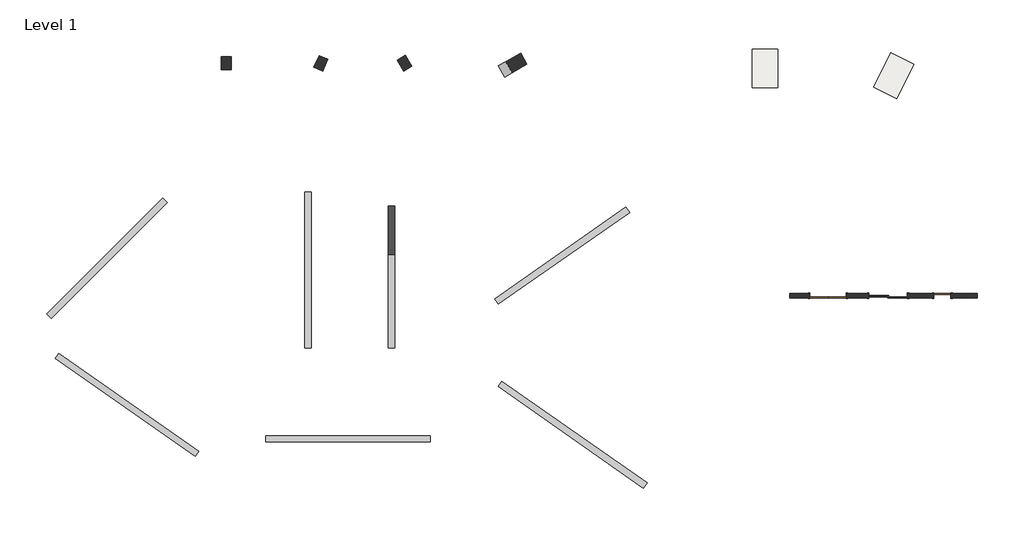
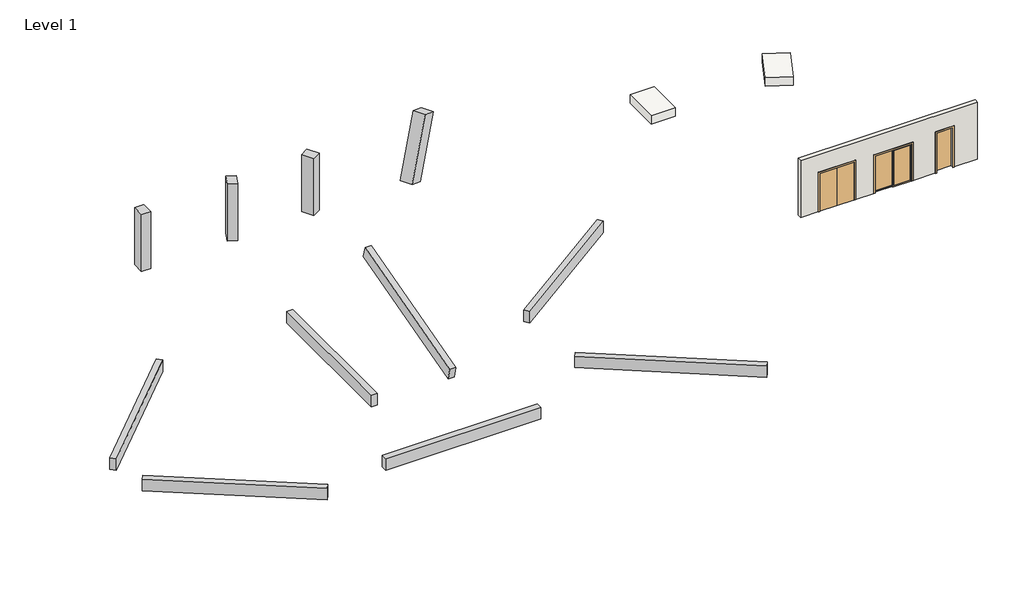
# One storey: 7 beams, 4 columns, 3 doors, 2 slabs, 1 wall.
"""IFC4 building model written with IfcOpenShell, lengths in millimetres."""

import ifcopenshell
import ifcopenshell.guid

model = None  # the IFC model being written
_history = None  # IfcOwnerHistory: only IFC2X3 demands one
_inside = {}  # id of a spatial element -> (the spatial element, [elements in it])
_under = {}  # id of a project, library or spatial element -> (it, [spatial elements below it])
_declared = {}  # id of a project -> (the project, [libraries it declares])
_typed = {}  # id of a type object -> (the type object, [elements of that type])
_made_of = {}  # id of a material, layer set ... -> (it, [elements and type objects made of it])


def new_model(schema):
    """Start an empty IFC model of exactly this schema.

    Asked for "IFC4X3", IfcOpenShell would pick the latest addendum, in which some entities
    have other attributes; the version numbers below select the first issue.
    IFC2X3 requires an IfcOwnerHistory on every rooted entity: one is made here for all.
    """
    global model, _history
    if schema == "IFC4X3":
        model = ifcopenshell.file(schema_version=(4, 3, 0, 0))
    else:
        model = ifcopenshell.file(schema=schema)
    _inside.clear()
    _under.clear()
    _declared.clear()
    _typed.clear()
    _made_of.clear()
    _history = None
    if model.schema == "IFC2X3":
        org = make("IfcOrganization", Name="unknown")
        user = make(
            "IfcPersonAndOrganization",
            ThePerson=make("IfcPerson", FamilyName="unknown"),
            TheOrganization=org,
        )
        app = make(
            "IfcApplication",
            ApplicationDeveloper=org,
            Version="unknown",
            ApplicationFullName="unknown",
            ApplicationIdentifier="unknown",
        )
        _history = make(
            "IfcOwnerHistory",
            OwningUser=user,
            OwningApplication=app,
            ChangeAction="ADDED",
            CreationDate=0,
        )
    return model


def make(cls, **values):
    """One entity of the class cls with the attributes given. An attribute that is None is left unset."""
    return model.create_entity(
        cls, **{name: value for name, value in values.items() if value is not None}
    )


def rooted(cls, **values):
    """An entity with a GlobalId (a new one), such as an element, a storey or a relation."""
    return make(cls, GlobalId=ifcopenshell.guid.new(), OwnerHistory=_history, **values)


def si_unit(unit_type, name, prefix=None):
    """IfcSIUnit, for example si_unit("LENGTHUNIT", "METRE", prefix="MILLI")."""
    return make("IfcSIUnit", UnitType=unit_type, Prefix=prefix, Name=name)


def assignment(units):
    """IfcUnitAssignment: the units of a project."""
    return None if units is None else make("IfcUnitAssignment", Units=units)


def point(xyz):
    """IfcCartesianPoint."""
    return None if xyz is None else make("IfcCartesianPoint", Coordinates=xyz)


def direction(xyz):
    """IfcDirection."""
    return None if xyz is None else make("IfcDirection", DirectionRatios=xyz)


def frame(location, z_axis=None, x_axis=None):
    """IfcAxis2Placement3D, a coordinate frame: its origin and axes. An axis left out is left unset."""
    return make(
        "IfcAxis2Placement3D",
        Location=point(location),
        Axis=direction(z_axis),
        RefDirection=direction(x_axis),
    )


def origin():
    """The frame at (0, 0, 0) with its axes left unset."""
    return frame((0.0, 0.0, 0.0))


def origin_with_axes():
    """The frame at (0, 0, 0) with the z axis (0, 0, 1) and the x axis (1, 0, 0) written out."""
    return frame((0.0, 0.0, 0.0), z_axis=(0.0, 0.0, 1.0), x_axis=(1.0, 0.0, 0.0))


def place(relative_to, where):
    """IfcLocalPlacement: puts the frame where relative to a parent placement (None: the world)."""
    return make(
        "IfcLocalPlacement", PlacementRelTo=relative_to, RelativePlacement=where
    )


def context(
    kind, dimensions, precision=None, world=None, true_north=None, identifier=None
):
    """IfcGeometricRepresentationContext, for example the 3D "Model" context."""
    return make(
        "IfcGeometricRepresentationContext",
        ContextIdentifier=identifier,
        ContextType=kind,
        CoordinateSpaceDimension=dimensions,
        Precision=precision,
        WorldCoordinateSystem=world,
        TrueNorth=true_north,
    )


def project(units=None, contexts=None):
    """IfcProject with its units and contexts."""
    return rooted(
        "IfcProject",
        Name="project",
        RepresentationContexts=contexts,
        UnitsInContext=assignment(units),
    )


def spatial(cls, under=None, at=None, **own):
    """A site, building, storey or space (cls), placed at a placement, below another one or the project."""
    s = rooted(cls, ObjectPlacement=at, **own)
    if under is not None:
        _under.setdefault(under.id(), (under, []))[1].append(s)
    return s


def polyline(points):
    """IfcPolyline through the points."""
    return make("IfcPolyline", Points=[point(p) for p in points])


def outline(outer, holes=None, kind="AREA"):
    """IfcArbitraryClosedProfileDef: a profile drawn as a closed curve; with holes, ...WithVoids."""
    if holes is None:
        return make("IfcArbitraryClosedProfileDef", ProfileType=kind, OuterCurve=outer)
    return make(
        "IfcArbitraryProfileDefWithVoids",
        ProfileType=kind,
        OuterCurve=outer,
        InnerCurves=holes,
    )


def extrude(swept, where, along, depth):
    """IfcExtrudedAreaSolid: the profile swept, set in the frame where, extruded along a direction by depth."""
    return make(
        "IfcExtrudedAreaSolid",
        SweptArea=swept,
        Position=where,
        ExtrudedDirection=direction(along),
        Depth=depth,
    )


def shape(context_of_items, identifier, shape_type, items):
    """IfcShapeRepresentation: the items that make up one representation, for example the "Body"."""
    return make(
        "IfcShapeRepresentation",
        ContextOfItems=context_of_items,
        RepresentationIdentifier=identifier,
        RepresentationType=shape_type,
        Items=items,
    )


def source(mapping_origin, context_of_items, identifier, shape_type, items):
    """IfcRepresentationMap: a shape defined once, which mapped items show again and again."""
    return make(
        "IfcRepresentationMap",
        MappingOrigin=mapping_origin,
        MappedRepresentation=shape(context_of_items, identifier, shape_type, items),
    )


def transform(
    local_origin,
    x_axis=None,
    y_axis=None,
    z_axis=None,
    scale=None,
    scale2=None,
    scale3=None,
    uniform=True,
):
    """IfcCartesianTransformationOperator3D, or its non-uniform kind. x_axis, y_axis, z_axis: its Axis1, 2, 3."""
    if uniform:
        return make(
            "IfcCartesianTransformationOperator3D",
            Axis1=direction(x_axis),
            Axis2=direction(y_axis),
            LocalOrigin=point(local_origin),
            Scale=scale,
            Axis3=direction(z_axis),
        )
    return make(
        "IfcCartesianTransformationOperator3DnonUniform",
        Axis1=direction(x_axis),
        Axis2=direction(y_axis),
        LocalOrigin=point(local_origin),
        Scale=scale,
        Axis3=direction(z_axis),
        Scale2=scale2,
        Scale3=scale3,
    )


def mapped(mapping_source, mapping_target):
    """IfcMappedItem: shows the shape of a source again, moved by a transform."""
    return make(
        "IfcMappedItem", MappingSource=mapping_source, MappingTarget=mapping_target
    )


def made_of(thing, what):
    """Note that an element or type object is made of a material, layer set ...; save() writes the relation."""
    if what is not None:
        _made_of.setdefault(what.id(), (what, []))[1].append(thing)
    return thing


def element(
    cls,
    number,
    at=None,
    inside=None,
    cuts=None,
    type_object=None,
    material=None,
    context=None,
    identifier="Body",
    shape_type=None,
    held_by="IfcProductDefinitionShape",
    body=None,
    shapes=None,
    **own,
):
    """One element of the class cls, such as IfcWall. Its Tag is "e" and its number.

    at: its placement. inside: the storey or other place that contains it. cuts: it is an
    opening in that element (IfcRelVoidsElement). A single representation is given by context,
    identifier, shape_type and body (its items); several are given by shapes. held_by: the class
    of the entity that holds the representations. save() writes the other relations.
    """
    e = rooted(cls, Tag="e%d" % number, ObjectPlacement=at, **own)
    if body is not None:
        shapes = [shape(context, identifier, shape_type, body)]
    if shapes is not None:
        e.Representation = make(held_by, Representations=shapes)
    if inside is not None:
        _inside.setdefault(inside.id(), (inside, []))[1].append(e)
    if cuts is not None:
        rooted(
            "IfcRelVoidsElement", RelatingBuildingElement=cuts, RelatedOpeningElement=e
        )
    if type_object is not None:
        _typed.setdefault(type_object.id(), (type_object, []))[1].append(e)
    return made_of(e, material)


def aggregate(whole, parts):
    """IfcRelAggregates: a whole, such as a stair, and the parts it consists of."""
    return rooted("IfcRelAggregates", RelatingObject=whole, RelatedObjects=parts)


def save(model, path):
    """Write the relations noted so far, then the file.

    IfcRelAggregates (storeys below a building ...), IfcRelContainedInSpatialStructure (elements
    in a storey), IfcRelDefinesByType, IfcRelAssociatesMaterial and IfcRelDeclares: one each for
    every whole, place, type object, material and project.
    """
    for whole, parts in _under.values():
        aggregate(whole, parts)
    for where, things in _inside.values():
        rooted(
            "IfcRelContainedInSpatialStructure",
            RelatedElements=things,
            RelatingStructure=where,
        )
    for kind, things in _typed.values():
        rooted("IfcRelDefinesByType", RelatedObjects=things, RelatingType=kind)
    for what, things in _made_of.values():
        rooted("IfcRelAssociatesMaterial", RelatedObjects=things, RelatingMaterial=what)
    for by, libraries in _declared.values():
        rooted("IfcRelDeclares", RelatingContext=by, RelatedDefinitions=libraries)
    model.write(path)


def concrete_rectangular_beam_300_x_600mm_0e8e550c(model_context):
    return source(origin(), model_context, "Body", "SweptSolid", [
        extrude(outline(polyline([(4000.0, 150.0), (4000.0, -150.0), (-4000.0, -150.0), (-4000.0, 150.0), (4000.0, 150.0)])), frame((0.0, 0.0, -300.0), z_axis=(0.0, 0.0, 1.0), x_axis=(1.0, 0.0, 0.0)), (0.0, 0.0, 1.0), 600.0),
    ])


def concrete_rectangular_beam_300_x_600mm_526adf45(model_context):
    return source(origin(), model_context, "Body", "SweptSolid", [
        extrude(outline(polyline([(3850.0, 150.0), (3850.0, -150.0), (-3850.0, -150.0), (-3850.0, 150.0), (3850.0, 150.0)])), frame((0.0, 0.0, -300.0), z_axis=(0.0, 0.0, 1.0), x_axis=(1.0, 0.0, 0.0)), (0.0, 0.0, 1.0), 600.0),
    ])


def concrete_rectangular_beam_300_x_600mm_2f98737b(model_context):
    return source(origin(), model_context, "Body", "SweptSolid", [
        extrude(outline(polyline([(3650.0, 150.0), (3650.0, -150.0), (-3650.0, -150.0), (-3650.0, 150.0), (3650.0, 150.0)])), frame((0.0, 0.0, -300.0), z_axis=(0.0, 0.0, 1.0), x_axis=(1.0, 0.0, 0.0)), (0.0, 0.0, 1.0), 600.0),
    ])


def concrete_rectangular_beam_300_x_600mm_b31908cc(model_context):
    return source(origin(), model_context, "Body", "SweptSolid", [
        extrude(outline(polyline([(3750.0, 150.0), (3750.0, -150.0), (-3750.0, -150.0), (-3750.0, 150.0), (3750.0, 150.0)])), frame((0.0, 0.0, -300.0), z_axis=(0.0, 0.0, 1.0), x_axis=(1.0, 0.0, 0.0)), (0.0, 0.0, 1.0), 600.0),
    ])


def concrete_rectangular_beam_300_x_600mm_b1d28744(model_context):
    return source(origin(), model_context, "Body", "SweptSolid", [
        extrude(outline(polyline([(4150.0, 150.0), (4150.0, -150.0), (-4150.0, -150.0), (-4150.0, 150.0), (4150.0, 150.0)])), frame((0.0, 0.0, -300.0), z_axis=(0.0, 0.0, 1.0), x_axis=(1.0, 0.0, 0.0)), (0.0, 0.0, 1.0), 600.0),
    ])


def concrete_rectangular_beam_300_x_600mm_07bb940a(model_context):
    return source(origin(), model_context, "Body", "SweptSolid", [
        extrude(outline(polyline([(3784.507894, 150.0), (3784.507894, -150.0), (-3784.507894, -150.0), (-3784.507894, 150.0), (3784.507894, 150.0)])), frame((0.0, 0.0, -300.0), z_axis=(0.0, 0.0, 1.0), x_axis=(1.0, 0.0, 0.0)), (0.0, 0.0, 1.0), 600.0),
    ])


def concrete_rectangular_column_450_x_600mm_2b408faa(model_context):
    return source(origin(), model_context, "Body", "SweptSolid", [
        extrude(outline(polyline([(225.0, 300.0), (225.0, -300.0), (-225.0, -300.0), (-225.0, 300.0), (225.0, 300.0)])), origin_with_axes(), (0.0, 0.0, 1.0), 3000.0),
    ])


def m_door_double_flush_panel_1700_x_2000mm_deeb3825(model_context):
    return source(origin(), model_context, "Body", "SweptSolid", [
        extrude(outline(polyline([(2000.0, -850.0), (2000.0, 850.0), (0.0, 850.0), (0.0, 930.0), (2080.0, 930.0), (2080.0, -930.0), (0.0, -930.0), (0.0, -850.0), (2000.0, -850.0)])), frame((0.0, -125.0, 0.0), z_axis=(0.0, 1.0, 0.0), x_axis=(0.0, 0.0, 1.0)), (0.0, 0.0, 1.0), 25.0),
        extrude(outline(polyline([(2000.0, -850.0), (2000.0, 850.0), (0.0, 850.0), (0.0, 930.0), (2080.0, 930.0), (2080.0, -930.0), (0.0, -930.0), (0.0, -850.0), (2000.0, -850.0)])), frame((0.0, 100.0, 0.0), z_axis=(0.0, 1.0, 0.0), x_axis=(0.0, 0.0, 1.0)), (0.0, 0.0, 1.0), 25.0),
        extrude(outline(polyline([(0.0, 100.0), (850.0, 100.0), (850.0, 50.0), (0.0, 50.0), (0.0, 100.0)])), origin_with_axes(), (0.0, 0.0, 1.0), 2000.0),
        extrude(outline(polyline([(-850.0, 100.0), (0.0, 100.0), (0.0, 50.0), (-850.0, 50.0), (-850.0, 100.0)])), origin_with_axes(), (0.0, 0.0, 1.0), 2000.0),
    ])


def m_door_double_sliding_1800_x_1950mm_ddb0fbbc(model_context):
    return source(origin(), model_context, "Body", "SweptSolid", [
        extrude(outline(polyline([(0.0, -980.0), (0.0, -900.0), (1950.0, -900.0), (1950.0, 900.0), (0.0, 900.0), (0.0, 980.0), (2030.0, 980.0), (2030.0, -980.0), (0.0, -980.0)])), frame((0.0, 2.0, 0.0), z_axis=(0.0, 1.0, 0.0), x_axis=(0.0, 0.0, 1.0)), (0.0, 0.0, 1.0), 25.0),
        extrude(outline(polyline([(0.0, 980.0), (2030.0, 980.0), (2030.0, -980.0), (0.0, -980.0), (0.0, -900.0), (1950.0, -900.0), (1950.0, 900.0), (0.0, 900.0), (0.0, 980.0)])), frame((0.0, 227.0, 0.0), z_axis=(0.0, 1.0, 0.0), x_axis=(0.0, 0.0, 1.0)), (0.0, 0.0, 1.0), 25.0),
        extrude(outline(polyline([(1950.0, -25.0), (0.0, -25.0), (0.0, 900.0), (1950.0, 900.0), (1950.0, -25.0)]), holes=[polyline([(1900.0, 25.0), (1900.0, 850.0), (50.0, 850.0), (50.0, 25.0), (1900.0, 25.0)])]), frame((0.0, 127.0, 0.0), z_axis=(0.0, 1.0, 0.0), x_axis=(0.0, 0.0, 1.0)), (0.0, 0.0, 1.0), 50.0),
        extrude(outline(polyline([(1950.0, 25.0), (1950.0, -900.0), (0.0, -900.0), (0.0, 25.0), (1950.0, 25.0)]), holes=[polyline([(1900.0, -25.0), (50.0, -25.0), (50.0, -850.0), (1900.0, -850.0), (1900.0, -25.0)])]), frame((0.0, 177.0, 0.0), z_axis=(0.0, 1.0, 0.0), x_axis=(0.0, 0.0, 1.0)), (0.0, 0.0, 1.0), 50.0),
        extrude(outline(polyline([(25.0, 155.175), (850.0, 155.175), (850.0, 148.825), (25.0, 148.825), (25.0, 155.175)])), frame((0.0, 0.0, 50.0), z_axis=(0.0, 0.0, 1.0), x_axis=(1.0, 0.0, 0.0)), (0.0, 0.0, 1.0), 1850.0),
        extrude(outline(polyline([(-25.0, 200.025), (-850.0, 200.025), (-850.0, 206.375), (-25.0, 206.375), (-25.0, 200.025)])), frame((0.0, 0.0, 50.0), z_axis=(0.0, 0.0, 1.0), x_axis=(1.0, 0.0, 0.0)), (0.0, 0.0, 1.0), 1850.0),
    ])


def m_door_single_panel_800_x_2100mm_e6cd55ec(model_context):
    return source(origin(), model_context, "Body", "SweptSolid", [
        extrude(outline(polyline([(400.0, 50.0), (-400.0, 50.0), (-400.0, 100.0), (400.0, 100.0), (400.0, 50.0)])), origin_with_axes(), (0.0, 0.0, 1.0), 2100.0),
        extrude(outline(polyline([(2176.2, -476.2), (0.0, -476.2), (0.0, -400.0), (2100.0, -400.0), (2100.0, 400.0), (0.0, 400.0), (0.0, 476.2), (2176.2, 476.2), (2176.2, -476.2)])), frame((0.0, 100.0, 0.0), z_axis=(0.0, 1.0, 0.0), x_axis=(0.0, 0.0, 1.0)), (0.0, 0.0, 1.0), 25.0),
        extrude(outline(polyline([(2176.2, 476.2), (2176.2, -476.2), (0.0, -476.2), (0.0, -400.0), (2100.0, -400.0), (2100.0, 400.0), (0.0, 400.0), (0.0, 476.2), (2176.2, 476.2)])), frame((0.0, -125.0, 0.0), z_axis=(0.0, 1.0, 0.0), x_axis=(0.0, 0.0, 1.0)), (0.0, 0.0, 1.0), 25.0),
    ])


def m_footing_rectangular_1800_x_1200_x_450mm_16ba7ea5(model_context):
    return source(origin(), model_context, "Body", "SweptSolid", [
        extrude(outline(polyline([(600.0, 900.0), (600.0, -900.0), (-600.0, -900.0), (-600.0, 900.0), (600.0, 900.0)])), frame((0.0, 0.0, -450.0), z_axis=(0.0, 0.0, 1.0), x_axis=(1.0, 0.0, 0.0)), (0.0, 0.0, 1.0), 450.0),
    ])


model = new_model("IFC4")

# Units and contexts
model_context = context("Model", 3, world=origin())
ifc_project = project(units=[si_unit("LENGTHUNIT", "METRE", prefix="MILLI")], contexts=[model_context])

# Site, building, storey
site = spatial("IfcSite", under=ifc_project)
building = spatial("IfcBuilding", under=site)
storey = spatial("IfcBuildingStorey", under=building, Name="Level 1", Elevation=0.0)

# Beams
placement = place(None, origin())
concrete_rectangular_beam_300_x_600mm_shape = concrete_rectangular_beam_300_x_600mm_0e8e550c(model_context)
element("IfcBeam", 1, ObjectType="Concrete-Rectangular Beam : 300 x 600mm", at=placement, inside=storey, context=model_context, shape_type="MappedRepresentation", body=[
    mapped(concrete_rectangular_beam_300_x_600mm_shape, transform((-9145.2085867, -16555.4936157, -300.0), x_axis=(0.8191520442889902, -0.5735764363510482, 0.0), y_axis=(0.5735764363510482, 0.8191520442889902, 0.0), z_axis=(0.0, 0.0, 1.0))),
])
concrete_rectangular_beam_300_x_600mm_2_shape = concrete_rectangular_beam_300_x_600mm_526adf45(model_context)
element("IfcBeam", 2, ObjectType="Concrete-Rectangular Beam : 300 x 600mm", at=placement, inside=storey, context=model_context, shape_type="MappedRepresentation", body=[
    mapped(concrete_rectangular_beam_300_x_600mm_2_shape, transform((-10087.4940608, -9679.7277386, -300.0), x_axis=(0.7071067811865487, 0.7071067811865464, 0.0), y_axis=(-0.7071067811865464, 0.7071067811865487, 0.0), z_axis=(0.0, 0.0, 1.0))),
])
element("IfcBeam", 3, ObjectType="Concrete-Rectangular Beam : 300 x 600mm", at=placement, inside=storey, context=model_context, shape_type="MappedRepresentation", body=[
    mapped(concrete_rectangular_beam_300_x_600mm_2_shape, transform((1194.8081303, -18143.0516491, -300.0), x_axis=(1.0, 0.0, 0.0), y_axis=(0.0, 1.0, 0.0), z_axis=(0.0, 0.0, 1.0))),
])
concrete_rectangular_beam_300_x_600mm_3_shape = concrete_rectangular_beam_300_x_600mm_2f98737b(model_context)
element("IfcBeam", 4, ObjectType="Concrete-Rectangular Beam : 300 x 600mm", at=placement, inside=storey, context=model_context, shape_type="MappedRepresentation", body=[
    mapped(concrete_rectangular_beam_300_x_600mm_3_shape, transform((-663.497906, -10225.1317807, -300.0), x_axis=(0.0, 1.0, 0.0), y_axis=(-1.0, 0.0, 0.0), z_axis=(0.0, 0.0, 1.0))),
])
concrete_rectangular_beam_300_x_600mm_4_shape = concrete_rectangular_beam_300_x_600mm_b31908cc(model_context)
element("IfcBeam", 5, ObjectType="Concrete-Rectangular Beam : 300 x 600mm", at=placement, inside=storey, context=model_context, shape_type="MappedRepresentation", body=[
    mapped(concrete_rectangular_beam_300_x_600mm_4_shape, transform((11230.4771438, -9556.8124673, -300.0), x_axis=(-0.8191520442889922, -0.5735764363510455, 0.0), y_axis=(0.5735764363510455, -0.8191520442889922, 0.0), z_axis=(0.0, 0.0, 1.0))),
])
concrete_rectangular_beam_300_x_600mm_5_shape = concrete_rectangular_beam_300_x_600mm_b1d28744(model_context)
element("IfcBeam", 6, ObjectType="Concrete-Rectangular Beam : 300 x 600mm", at=placement, inside=storey, context=model_context, shape_type="MappedRepresentation", body=[
    mapped(concrete_rectangular_beam_300_x_600mm_5_shape, transform((11724.551203, -17950.7315453, -300.0), x_axis=(-0.8191520442889885, 0.5735764363510507, 0.0), y_axis=(-0.5735764363510507, -0.8191520442889885, 0.0), z_axis=(0.0, 0.0, 1.0))),
])
concrete_rectangular_beam_300_x_600mm_6_shape = concrete_rectangular_beam_300_x_600mm_07bb940a(model_context)
element("IfcBeam", 7, ObjectType="Concrete-Rectangular Beam : 300 x 600mm", at=placement, inside=storey, context=model_context, shape_type="MappedRepresentation", body=[
    mapped(concrete_rectangular_beam_300_x_600mm_6_shape, transform((3236.502094, -10145.8612366, 710.6625139), x_axis=(0.0, 0.9644582868368909, 0.2642351470786003), y_axis=(-1.0, 0.0, 0.0), z_axis=(0.0, -0.2642351470786003, 0.9644582868368909))),
])

# Columns
concrete_rectangular_column_450_x_600mm_shape = concrete_rectangular_column_450_x_600mm_2b408faa(model_context)
element("IfcColumn", 8, ObjectType="Concrete-Rectangular-Column : 450 x 600mm", at=placement, inside=storey, context=model_context, shape_type="MappedRepresentation", body=[
    mapped(concrete_rectangular_column_450_x_600mm_shape, transform((-4498.8166129, -540.542419, 0.0), x_axis=(1.0, 0.0, 0.0), y_axis=(0.0, 1.0, 0.0), z_axis=(0.0, 0.0, 1.0))),
])
element("IfcColumn", 9, ObjectType="Concrete-Rectangular-Column : 450 x 600mm", at=placement, inside=storey, context=model_context, shape_type="MappedRepresentation", body=[
    mapped(concrete_rectangular_column_450_x_600mm_shape, transform((-64.8783295, -540.542419, 0.0), x_axis=(0.9135454576425981, -0.40673664307580637, 0.0), y_axis=(0.40673664307580637, 0.9135454576425981, 0.0), z_axis=(0.0, 0.0, 1.0))),
])
element("IfcColumn", 10, ObjectType="Concrete-Rectangular-Column : 450 x 600mm", at=placement, inside=storey, context=model_context, shape_type="MappedRepresentation", body=[
    mapped(concrete_rectangular_column_450_x_600mm_shape, transform((3848.4631718, -540.542419, 0.0), x_axis=(0.8571673007021157, 0.5150380749100485, 0.0), y_axis=(-0.5150380749100485, 0.8571673007021157, 0.0), z_axis=(0.0, 0.0, 1.0))),
])
element("IfcColumn", 11, ObjectType="Concrete-Rectangular-Column : 600 x 750mm", at=placement, inside=storey, context=model_context, shape_type="SweptSolid", body=[
    extrude(outline(polyline([(600.0, 0.0), (600.0, -750.0), (0.0, -750.0), (0.0, 0.0), (600.0, 0.0)])), frame((8541.7495915, -1181.0366975, 130.4944773), z_axis=(0.30136408628102856, 0.17399263633843867, 0.9375000000000002), x_axis=(-0.5000000000000028, 0.866025403784437, 0.0)), (0.0, 0.0, 1.0), 3200.0),
])

# Doors
m_door_double_flush_panel_1700_x_2000mm_shape = m_door_double_flush_panel_1700_x_2000mm_deeb3825(model_context)
element("IfcDoor", 12, ObjectType="M_Door-Double-Flush_Panel : 1700 x 2000mm", at=placement, inside=storey, context=model_context, shape_type="MappedRepresentation", body=[
    mapped(m_door_double_flush_panel_1700_x_2000mm_shape, transform((23681.5621943, -11433.3538056, 0.0), x_axis=(-1.0, 0.0, 0.0), y_axis=(0.0, -1.0, 0.0), z_axis=(0.0, 0.0, 1.0))),
])
m_door_double_sliding_1800_x_1950mm_shape = m_door_double_sliding_1800_x_1950mm_ddb0fbbc(model_context)
element("IfcDoor", 13, ObjectType="M_Door-Double-Sliding : 1800 x 1950mm", at=placement, inside=storey, context=model_context, shape_type="MappedRepresentation", body=[
    mapped(m_door_double_sliding_1800_x_1950mm_shape, transform((26491.5621943, -11306.3538056, 0.0), x_axis=(-1.0, 0.0, 0.0), y_axis=(0.0, -1.0, 0.0), z_axis=(0.0, 0.0, 1.0))),
])
m_door_single_panel_800_x_2100mm_shape = m_door_single_panel_800_x_2100mm_e6cd55ec(model_context)
element("IfcDoor", 14, ObjectType="M_Door-Single-Panel : 800 x 2100mm", at=placement, inside=storey, context=model_context, shape_type="MappedRepresentation", body=[
    mapped(m_door_single_panel_800_x_2100mm_shape, transform((29036.5621943, -11433.3538056, 0.0), x_axis=(1.0, 0.0, 0.0), y_axis=(0.0, 1.0, 0.0), z_axis=(0.0, 0.0, 1.0))),
])

# Slabs
m_footing_rectangular_1800_x_1200_x_450mm_shape = m_footing_rectangular_1800_x_1200_x_450mm_16ba7ea5(model_context)
element("IfcSlab", 15, ObjectType="M_Footing-Rectangular : 1800 x 1200 x 450mm", at=placement, inside=storey, context=model_context, shape_type="MappedRepresentation", body=[
    mapped(m_footing_rectangular_1800_x_1200_x_450mm_shape, transform((20736.502094, -775.1317807, 0.0), x_axis=(1.0, 0.0, 0.0), y_axis=(0.0, 1.0, 0.0), z_axis=(0.0, 0.0, 1.0))),
])
element("IfcSlab", 16, ObjectType="M_Footing-Rectangular : 1800 x 1200 x 450mm", at=placement, inside=storey, context=model_context, shape_type="MappedRepresentation", body=[
    mapped(m_footing_rectangular_1800_x_1200_x_450mm_shape, transform((26762.5678616, -1118.6772691, 0.0), x_axis=(0.898794046299165, -0.4383711467890819, 0.0), y_axis=(0.4383711467890819, 0.898794046299165, 0.0), z_axis=(0.0, 0.0, 1.0))),
])

# Wall
element("IfcWall", 17, ObjectType="Generic - 200mm", at=placement, inside=storey, context=model_context, shape_type="SweptSolid", body=[
    extrude(outline(polyline([(2100.0, 29436.5621943), (0.0, 29436.5621943), (0.0, 30676.5621943), (3000.0, 30676.5621943), (3000.0, 21876.5621943), (0.0, 21876.5621943), (0.0, 22831.5621943), (2000.0, 22831.5621943), (2000.0, 24531.5621943), (0.0, 24531.5621943), (0.0, 25591.5621943), (1950.0, 25591.5621943), (1950.0, 27391.5621943), (0.0, 27391.5621943), (0.0, 28636.5621943), (2100.0, 28636.5621943), (2100.0, 29436.5621943)])), frame((0.0, -11533.3538056, 0.0), z_axis=(0.0, 1.0, 0.0), x_axis=(0.0, 0.0, 1.0)), (0.0, 0.0, 1.0), 200.0),
])

save(model, "model.ifc")

# Revit data of these elements
# Project information
#   Project Issue Date = "Issue Date"
#   Project Status = "Project Status"
#   Client Name = "Owner"
#   Project Address = "Enter address here"
#   Project Name = "Project Name"
#   Project Number = "Project Number"
#   SR Document GUID = "d4a11de3-9f94-4c30-a072-1203588bd18a"
# Type "Concrete-Rectangular Beam : 300 x 600mm"
#   Length [instance default] = 1524 mm
#   b = 300 mm
#   h = 600 mm
#   Structural Material [instance default] = Concrete, Cast-in-Place gray
#   Assembly Code = ""
# Type "Concrete-Rectangular-Column : 450 x 600mm"
#   b = 450 mm
#   h = 600 mm
#   Structural Material [instance default] = none
# Type "Concrete-Rectangular-Column : 600 x 750mm"
#   b = 600 mm
#   h = 750 mm
#   Structural Material [instance default] = none
# Type "M_Door-Double-Flush_Panel : 1700 x 2000mm"
#   Type Mark = "41"
#   Construction Type Id = "DOOR"
#   Assembly Code = "C1020"
#   Analytic Construction = "Wooden"
#   Thickness = 50 mm
#   Thermal Resistance (R) = 0.455703 (m²·K)/W
#   Swing Angle [instance default] = 90.00°
#   Panel Width = 850 mm
#   Heat Transfer Coefficient (U) = 2.19465 W/(m²·K)
#   Height = 2000 mm
#   Trim Projection Ext = 25 mm
#   Trim Projection Int = 25 mm
#   Trim Width = 80 mm
#   Width = 1700 mm
#   Panel Material = Wood - Birch - Solid Stained Light Low Gloss
#   Trim Material = Paint - Sienna
#   Visual Light Transmittance = 0
#   Solar Heat Gain Coefficient = 0
#   Function = (empty or 0)
#   Wall Closure = (empty or 0)
# Type "M_Door-Double-Sliding : 1800 x 1950mm"
#   Type Mark = "42"
#   Construction Type Id = "opn-d45"
#   Assembly Code = "C1020"
#   Analytic Construction = "Wood frame, double glass door "
#   Thickness = 50 mm
#   Thermal Resistance (R) = 0.31964 (m²·K)/W
#   Heat Transfer Coefficient (U) = 3.12872 W/(m²·K)
#   Height = 1950 mm
#   Rail Width = 50 mm
#   Stiles = 50 mm
#   Trim Projection Ext = 25 mm
#   Trim Projection Int = 25 mm
#   Trim Width = 80 mm
#   Width = 1800 mm
#   Glazing = Glass
#   Panel Material = Wood - Birch - Solid Stained Light Low Gloss
#   Trim Material = Paint - Sienna
#   Visual Light Transmittance = 0
#   Solar Heat Gain Coefficient = 0
#   Function = (empty or 0)
#   Wall Closure = (empty or 0)
# Type "M_Door-Single-Panel : 800 x 2100mm"
#   Type Mark = "43"
#   Construction Type Id = "DOOR"
#   Assembly Code = "C1020300"
#   Analytic Construction = "Wooden"
#   Thickness = 50 mm
#   Thermal Resistance (R) = 0.455703 (m²·K)/W
#   Swing Angle [instance default] = 90.00°
#   Heat Transfer Coefficient (U) = 2.19465 W/(m²·K)
#   Height = 2100 mm
#   Trim Projection Ext = 25 mm
#   Trim Projection Int = 25 mm
#   Trim Width = 80 mm
#   Width = 800 mm
#   Panel Material = Wood - Birch - Solid Stained Light Low Gloss
#   Trim Material = Paint - Sienna
#   Visual Light Transmittance = 0
#   Solar Heat Gain Coefficient = 0
#   Function = (empty or 0)
#   Wall Closure = (empty or 0)
# Type "M_Footing-Rectangular : 1800 x 1200 x 450mm"
#   Width = 1200 mm
#   Length = 1800 mm
#   Thickness = 450 mm
#   Structural Material [instance default] = none
#   Assembly Code = ""
# Type "Generic - 200mm"
#   Layers, outside or top first: 200 mm no material (function 1)
# Element 1 (IfcBeam, "Concrete-Rectangular Beam : 300 x 600mm")
#   Mark = "B2"
#   Structural Material = Concrete, Cast-in-Place gray
#   Phase Created = New Construction
#   Materials on its faces: "Concrete, Cast-in-Place gray"
# Element 2 (IfcBeam, "Concrete-Rectangular Beam : 300 x 600mm")
#   Mark = "B1"
#   Structural Material = Concrete, Cast-in-Place gray
#   Phase Created = New Construction
#   Materials on its faces: "Concrete, Cast-in-Place gray"
# Element 3 (IfcBeam, "Concrete-Rectangular Beam : 300 x 600mm")
#   Mark = "B3"
#   Structural Material = Concrete, Cast-in-Place gray
#   Phase Created = New Construction
#   Materials on its faces: "Concrete, Cast-in-Place gray"
# Element 4 (IfcBeam, "Concrete-Rectangular Beam : 300 x 600mm")
#   Mark = "B4"
#   Structural Material = Concrete, Cast-in-Place gray
#   Phase Created = New Construction
#   Materials on its faces: "Concrete, Cast-in-Place gray"
# Element 5 (IfcBeam, "Concrete-Rectangular Beam : 300 x 600mm")
#   Mark = "B6"
#   Structural Material = Concrete, Cast-in-Place gray
#   Phase Created = New Construction
#   Materials on its faces: "Concrete, Cast-in-Place gray"
# Element 6 (IfcBeam, "Concrete-Rectangular Beam : 300 x 600mm")
#   Mark = "B7"
#   Structural Material = Concrete, Cast-in-Place gray
#   Phase Created = New Construction
#   Materials on its faces: "Concrete, Cast-in-Place gray"
# Element 7 (IfcBeam, "Concrete-Rectangular Beam : 300 x 600mm")
#   Mark = "B5"
#   Structural Material = Concrete, Cast-in-Place gray
#   Phase Created = New Construction
#   Materials on its faces: "Concrete, Cast-in-Place gray"
# Element 8 (IfcColumn, "Concrete-Rectangular-Column : 450 x 600mm")
#   Mark = "C1"
#   Structural Material = Concrete - Cast-in-Place Concrete - C30/37
#   Phase Created = New Construction
#   Materials on its faces: "Concrete - Cast-in-Place Concrete - C30/37"
# Element 9 (IfcColumn, "Concrete-Rectangular-Column : 450 x 600mm")
#   Mark = "C2"
#   Structural Material = Concrete - Cast-in-Place Concrete - C30/37
#   Phase Created = New Construction
#   Materials on its faces: "Concrete - Cast-in-Place Concrete - C30/37"
# Element 10 (IfcColumn, "Concrete-Rectangular-Column : 450 x 600mm")
#   Mark = "C3"
#   Structural Material = Concrete - Cast-in-Place Concrete - C30/37
#   Phase Created = New Construction
#   Materials on its faces: "Concrete - Cast-in-Place Concrete - C30/37"
# Element 11 (IfcColumn, "Concrete-Rectangular-Column : 600 x 750mm")
#   Mark = "C4"
#   Structural Material = Concrete - Cast-in-Place Concrete - C30/37
#   Phase Created = New Construction
#   Materials on its faces: "Concrete - Cast-in-Place Concrete - C30/37"
# Element 12 (IfcDoor, "M_Door-Double-Flush_Panel : 1700 x 2000mm")
#   Phase Created = New Construction
#   Materials on its faces: "Paint - Sienna", "Wood - Birch - Solid Stained Light Low Gloss"
# Element 13 (IfcDoor, "M_Door-Double-Sliding : 1800 x 1950mm")
#   Phase Created = New Construction
#   Materials on its faces: "Paint - Sienna", "Wood - Birch - Solid Stained Light Low Gloss", "Glass"
# Element 14 (IfcDoor, "M_Door-Single-Panel : 800 x 2100mm")
#   Phase Created = New Construction
#   Materials on its faces: "Paint - Sienna", "Wood - Birch - Solid Stained Light Low Gloss"
# Element 15 (IfcSlab, "M_Footing-Rectangular : 1800 x 1200 x 450mm")
#   Mark = "GM1"
#   Structural Material = none
#   Phase Created = New Construction
# Element 16 (IfcSlab, "M_Footing-Rectangular : 1800 x 1200 x 450mm")
#   Mark = "GM2"
#   Structural Material = none
#   Phase Created = New Construction
# Element 17 (IfcWall, "Generic - 200mm")
#   Comments = ""
#   Top Offset = 0 mm
#   Base Offset = 0 mm
#   wall height = 3000 mm
#   Phase Created = New Construction
#   Base Constraint = Level 1
#   Top Constraint = Level 2
#   Materials on its faces: "Default Wall"
# Materials
#   "Concrete, Cast-in-Place gray": class "Concrete", colour RGB 192 192 192, transparency 0, Description = "Cast-in-place concrete", Cost = 0
#   "Wood - Birch - Solid Stained Light Low Gloss": class "Wood", colour RGB 210 159 95, transparency 0, Cost = 0
#   "Paint - Sienna": class "Miscellaneous", colour RGB 118 70 51, transparency 0, Cost = 0
#   "Glass": class "Glass", colour RGB 55 55 255, transparency 0.9, Description = "Soda Lime Glass", Cost = 0
#   "Concrete - Cast-in-Place Concrete - C30/37": class "Unassigned", colour RGB 192 192 192, transparency 0
#   "Default Wall": class "Unassigned", colour RGB 128 128 128, transparency 0
